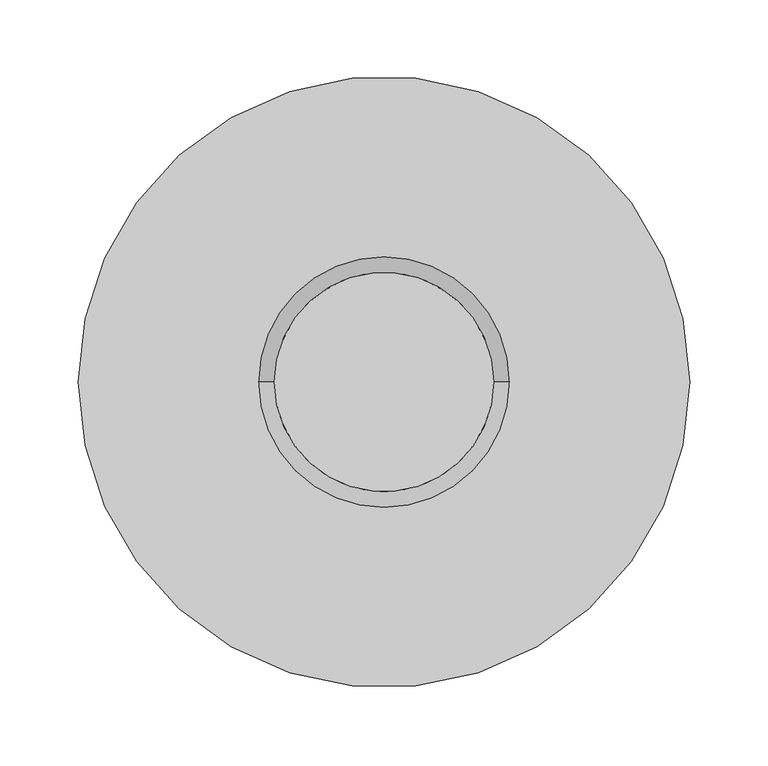
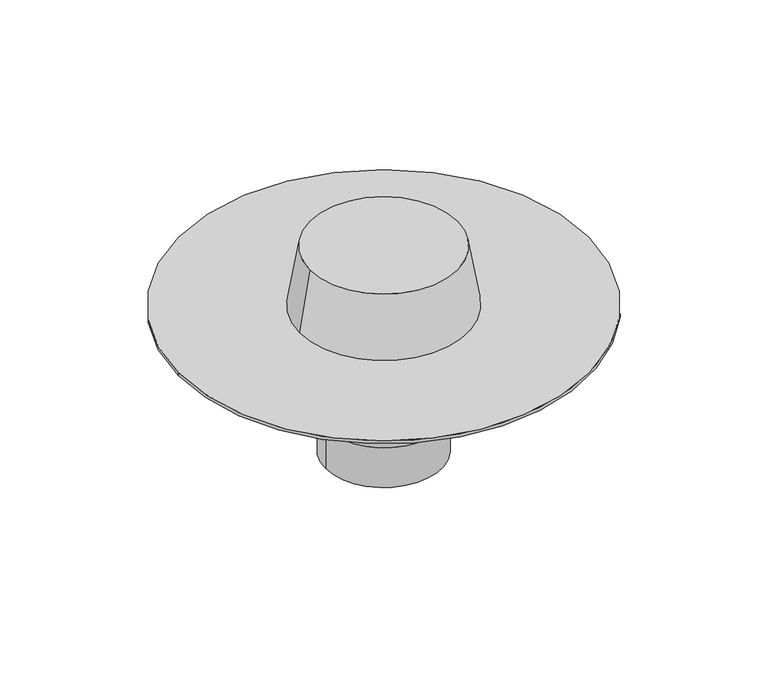
"""IFC4 building model written with IfcOpenShell, lengths in millimetres: proxy geometry, TN_Воронка ТехноНИКОЛЬ ВБ : Воронка ТехноНИКОЛЬ ВБ ЭКО, 110х145."""

from ifc_helpers import new_model, si_unit, point, frame, origin, origin_2d, place, context, project, spatial, polyline, circle_curve, trimmed, segment, composite_curve, outline, extrude, source, transform, mapped, element, save
from ifc_brep_helpers import plane_surface, revolved_surface, advanced_brep


def specialty_equipment_fe572f6f(model_context):
    return source(origin(), model_context, "Body", "SolidModel", [
        advanced_brep(
        [(70.0, 0.0, -85.0), (-70.0, 0.0, -85.0), (55.0, 0.0, -105.0), (-55.0, 0.0, -105.0)],
        [
            (0, 1, circle_curve(frame((0.0, 0.0, -85.0), z_axis=(0.0, 0.0, 1.0), x_axis=(1.0, 0.0, 0.0)), 70.0)),
            (1, 0, circle_curve(frame((0.0, 0.0, -85.0), z_axis=(0.0, 0.0, 1.0), x_axis=(-1.0, 0.0, 0.0)), 70.0)),
            (2, 3, circle_curve(frame((0.0, 0.0, -105.0), z_axis=(0.0, 0.0, -1.0), x_axis=(-1.0, 0.0, 0.0)), 55.0)),
            (3, 2, circle_curve(frame((0.0, 0.0, -105.0), z_axis=(0.0, 0.0, -1.0), x_axis=(1.0, 0.0, 0.0)), 55.0)),
            (3, 1),
            (0, 2),
        ],
        [
            plane_surface(frame((0.0, 0.0, -85.0), z_axis=(0.0, 0.0, 1.0), x_axis=(0.0, 1.0, 0.0))),
            plane_surface(frame((0.0, 0.0, -105.0), z_axis=(0.0, 0.0, -1.0), x_axis=(0.0, 1.0, 0.0))),
            revolved_surface(polyline([(-54.99999999464286, 0.0, -105.0), (-70.0, 0.0, -85.0)]), (0.0, 0.0, -178.3333333), (0.0, 0.0, 1.0)),
            revolved_surface(polyline([(54.99999999464286, 0.0, -105.0), (70.0, 0.0, -85.0)]), (0.0, 0.0, -178.3333333), (0.0, 0.0, 1.0)),
        ],
        [
            (0, [[1, 2]]),
            (1, [[3, 4]]),
            (2, [[-4, 5, -1, 6]]),
            (3, [[-3, -6, -2, -5]]),
        ],
    ),
        extrude(outline(composite_curve([segment(trimmed(circle_curve(origin_2d(), 70.0), [point((-70.0, 0.0))], [point((70.0, 0.0))], False, "CARTESIAN"), True, "CONTINUOUS"), segment(trimmed(circle_curve(origin_2d(), 70.0), [point((70.0, 0.0))], [point((-70.0, 0.0))], False, "CARTESIAN"), True, "CONTINUOUS")], self_intersect=False)), frame((0.0, 0.0, -85.0), z_axis=(0.0, 0.0, 1.0), x_axis=(1.0, 0.0, 0.0)), (0.0, 0.0, 1.0), 82.0),
        extrude(outline(composite_curve([segment(trimmed(circle_curve(origin_2d(), 55.0), [point((55.0, 0.0))], [point((-55.0, 0.0))], False, "CARTESIAN"), True, "CONTINUOUS"), segment(trimmed(circle_curve(origin_2d(), 55.0), [point((-55.0, 0.0))], [point((55.0, 0.0))], False, "CARTESIAN"), True, "CONTINUOUS")], self_intersect=False)), frame((0.0, 0.0, -145.0), z_axis=(0.0, 0.0, 1.0), x_axis=(1.0, 0.0, 0.0)), (0.0, 0.0, 1.0), 40.0),
        extrude(outline(composite_curve([segment(trimmed(circle_curve(origin_2d(), 195.0), [point((-195.0, 0.0))], [point((195.0, 0.0))], False, "CARTESIAN"), True, "CONTINUOUS"), segment(trimmed(circle_curve(origin_2d(), 195.0), [point((195.0, 0.0))], [point((-195.0, 0.0))], False, "CARTESIAN"), True, "CONTINUOUS")], self_intersect=False)), frame((0.0, 0.0, -3.0), z_axis=(0.0, 0.0, 1.0), x_axis=(1.0, 0.0, 0.0)), (0.0, 0.0, 1.0), 3.0),
        advanced_brep(
        [(-70.0, 0.0, 60.0), (70.0, 0.0, 60.0), (-80.0, 0.0, 0.0), (80.0, 0.0, 0.0)],
        [
            (0, 1, circle_curve(frame((0.0, 0.0, 60.0), z_axis=(0.0, 0.0, 1.0), x_axis=(-1.0, 0.0, 0.0)), 70.0)),
            (1, 0, circle_curve(frame((0.0, 0.0, 60.0), z_axis=(0.0, 0.0, 1.0), x_axis=(1.0, 0.0, 0.0)), 70.0)),
            (2, 3, circle_curve(frame((0.0, 0.0, 0.0), z_axis=(0.0, 0.0, -1.0), x_axis=(1.0, 0.0, 0.0)), 80.0)),
            (3, 2, circle_curve(frame((0.0, 0.0, 0.0), z_axis=(0.0, 0.0, -1.0), x_axis=(-1.0, 0.0, 0.0)), 80.0)),
            (3, 1),
            (0, 2),
        ],
        [
            plane_surface(frame((0.0, 0.0, 60.0), z_axis=(0.0, 0.0, 1.0), x_axis=(0.0, -1.0, 0.0))),
            plane_surface(frame((0.0, 0.0, 0.0), z_axis=(0.0, 0.0, -1.0), x_axis=(0.0, -1.0, 0.0))),
            revolved_surface(polyline([(-70.0, 0.0, 60.0), (-80.0, 0.0, 0.0)]), (0.0, 0.0, 480.0), (0.0, 0.0, -1.0)),
            revolved_surface(polyline([(70.0, 0.0, 60.0), (80.0, 0.0, 0.0)]), (0.0, 0.0, 480.0), (0.0, 0.0, -1.0)),
        ],
        [
            (0, [[1, 2]]),
            (1, [[3, 4]]),
            (2, [[-4, 5, -1, 6]]),
            (3, [[-3, -6, -2, -5]]),
        ],
    ),
    ])


if __name__ == "__main__":
    model = new_model("IFC4")
    model_context = context("Model", 3, world=origin())
    ifc_project = project(units=[si_unit("LENGTHUNIT", "METRE", prefix="MILLI")], contexts=[model_context])
    site = spatial("IfcSite", under=ifc_project)
    building = spatial("IfcBuilding", under=site)
    placement = place(None, origin())
    specialty_equipment_shape = specialty_equipment_fe572f6f(model_context)
    element("IfcBuildingElementProxy", 1, Name="TN_Воронка ТехноНИКОЛЬ ВБ : Воронка ТехноНИКОЛЬ ВБ ЭКО, 110х145", ObjectType="TN_Воронка ТехноНИКОЛЬ ВБ : Воронка ТехноНИКОЛЬ ВБ ЭКО, 110х145", at=placement, inside=building, context=model_context, shape_type="MappedRepresentation", body=[
        mapped(specialty_equipment_shape, transform((0.0, 0.0, 0.0), x_axis=(1.0, 0.0, 0.0), y_axis=(0.0, 1.0, 0.0), z_axis=(0.0, 0.0, 1.0))),
    ])
    save(model, "model.ifc")

# Revit data of these elements
# Type "TN_Воронка ТехноНИКОЛЬ ВБ : Воронка ТехноНИКОЛЬ ВБ ЭКО, 110х145"
#   ADSK_Группирование = "Комплектующие и воронки"
#   Description = "Кровельные воронки ТехноНИКОЛЬ ВБ ЭКО 110х145 применяются для организации внутреннего водостока с плоских кровель. Воронки могут устанавливаться в кровлю безогневым способом на мастику герметизирующую № 71. Воронки ТехноНИКОЛЬ ВБ ЭКО 110х145 используются при ремонте и строительстве зданий и сооружений с плоскими кровлями. Применяются в кровлях из битумных и битумнополимерных рулонных и мастичных материалов с внутренним водостоком. Количество воронок определяется расчетом. Пропуская способность 7,8 л/сек."
#   Manufacturer = "ТехноНИКОЛЬ"
#   URL = "https://shop.tn.ru/voronka-tehnonikol-vb-jeko-110h145-mm"
#   ADSK_Примечание = ""
#   ADSK_Обозначение = "ТехноНИКОЛЬ"
#   ADSK_Наименование = "Воронка ТехноНИКОЛЬ ВБ ЭКО, 110х145"
#   ADSK_Марка = ""
#   ADSK_Код изделия = "460065"
#   ADSK_Завод-изготовитель = "ТехноНИКОЛЬ"
#   ADSK_Единица измерения = "шт."
#   ADSK_Группирование = "Комплектующие и воронки"
#   ADSK_URL страницы изделия = "https://shop.tn.ru/voronka-tehnonikol-vb-jeko-110h145-mm"
#   ADSK_URL документации изделия = "https://nav.tn.ru/catalog/krovlya/vodostochnaya-sistema/voronka-tekhnonikol-vb-eko/?sphrase_id=114614"
#   Диаметр фланца = 390 mm
#   Высота воронки = 145 mm
#   ADSK_Масса = 0.58
#   ADSK_Количество = 1
#   Материал = TN_ПВХ_Черный
#   Default Elevation = 0
# Element 1 (IfcBuildingElementProxy, "TN_Воронка ТехноНИКОЛЬ ВБ : Воронка ТехноНИКОЛЬ ВБ ЭКО, 110х145")
#   Materials on its faces: "TN_ПВХ_Черный"
# Materials
#   "TN_ПВХ_Черный": class "Типовые", colour RGB 48 48 48, transparency 0, Cost = 0
